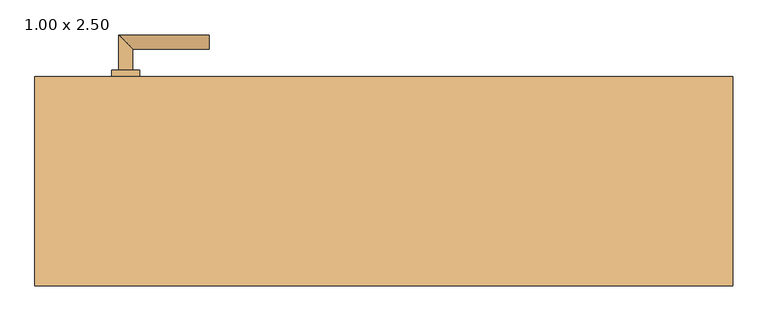
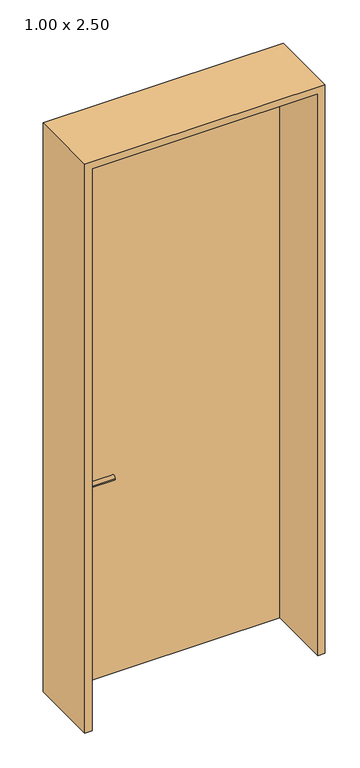
"""IFC4 building model written with IfcOpenShell, lengths in millimetres: door geometry, Drehflügel 1-flg - Blockzarge : 1.00 x 2.50."""

from ifc_helpers import new_model, si_unit, point, frame, frame_2d, origin, place, context, project, spatial, polyline, circle_curve, ellipse_curve, trimmed, segment, composite_curve, outline, extrude, source, transform, mapped, element, save
from ifc_brep_helpers import plane_surface, cylinder_surface, advanced_brep


def door_1_00_x_2_50_427c85ad(model_context):
    return source(origin(), model_context, "Body", "SolidModel", [
        advanced_brep(
        [(-360.0, 129.4346141, 1000.0), (-380.0, 129.4346141, 1000.0), (-360.0, 99.4346141, 1000.0), (-380.0, 79.4346141, 1000.0), (-250.0, 99.4346141, 1000.0), (-250.0, 79.4346141, 1000.0)],
        [
            (0, 1, circle_curve(frame((-370.0, 129.4346141, 1000.0), z_axis=(0.0, 1.0, 0.0), x_axis=(-1.0, 0.0, 0.0)), 10.0)),
            (1, 0, circle_curve(frame((-370.0, 129.4346141, 1000.0), z_axis=(0.0, 1.0, 0.0), x_axis=(-1.0, 0.0, 0.0)), 10.0)),
            (0, 2),
            (2, 3, ellipse_curve(frame((-370.0, 89.4346141, 1000.0), z_axis=(-0.7071067811865686, 0.7071067811865265, 0.0), x_axis=(0.7071067811865264, 0.7071067811865687, 0.0)), 14.1421356, 10.0)),
            (3, 1),
            (3, 2, ellipse_curve(frame((-370.0, 89.4346141, 1000.0), z_axis=(-0.7071067811865686, 0.7071067811865265, 0.0), x_axis=(0.7071067811865264, 0.7071067811865687, 0.0)), 14.1421356, 10.0)),
            (4, 5, circle_curve(frame((-250.0, 89.4346141, 1000.0), z_axis=(1.0, 0.0, 0.0), x_axis=(0.0, -1.0, 0.0)), 10.0)),
            (5, 4, circle_curve(frame((-250.0, 89.4346141, 1000.0), z_axis=(1.0, 0.0, 0.0), x_axis=(0.0, -1.0, 0.0)), 10.0)),
            (2, 4),
            (5, 3),
        ],
        [
            plane_surface(frame((-370.0, 129.4346141, -287.7526403), z_axis=(0.0, 1.0, 0.0), x_axis=(0.0, 0.0, 1.0))),
            cylinder_surface(frame((-370.0, 129.4346141, 1000.0), z_axis=(0.0, 1.0, 0.0), x_axis=(-1.0, 0.0, 0.0)), 10.0),
            plane_surface(frame((-250.0, 89.4346141, -287.7526403), z_axis=(1.0, 0.0, 0.0), x_axis=(0.0, 0.0, 1.0))),
            cylinder_surface(frame((-370.0, 89.4346141, 1000.0), z_axis=(-1.0, 0.0, 0.0), x_axis=(0.0, -1.0, 0.0)), 10.0),
        ],
        [
            (0, [[1, 2]]),
            (1, [[-1, 3, 4, 5]]),
            (1, [[-2, -5, 6, -3]]),
            (2, [[7, 8]]),
            (3, [[-4, 9, -8, 10]]),
            (3, [[-6, -10, -7, -9]]),
        ],
    ),
        advanced_brep(
        [(-360.0, 174.4346141, 1000.0), (-380.0, 174.4346141, 1000.0), (-360.0, 204.4346141, 1000.0), (-380.0, 224.4346141, 1000.0), (-250.0, 204.4346141, 1000.0), (-250.0, 224.4346141, 1000.0)],
        [
            (0, 1, circle_curve(frame((-370.0, 174.4346141, 1000.0), z_axis=(0.0, -1.0, 0.0), x_axis=(-1.0, 0.0, 0.0)), 10.0)),
            (1, 0, circle_curve(frame((-370.0, 174.4346141, 1000.0), z_axis=(0.0, -1.0, 0.0), x_axis=(-1.0, 0.0, 0.0)), 10.0)),
            (0, 2),
            (2, 3, ellipse_curve(frame((-370.0, 214.4346141, 1000.0), z_axis=(-0.7071067811865486, -0.7071067811865464, 0.0), x_axis=(0.7071067811865464, -0.7071067811865488, 0.0)), 14.1421356, 10.0)),
            (3, 1),
            (3, 2, ellipse_curve(frame((-370.0, 214.4346141, 1000.0), z_axis=(-0.7071067811865486, -0.7071067811865464, 0.0), x_axis=(0.7071067811865464, -0.7071067811865488, 0.0)), 14.1421356, 10.0)),
            (4, 5, circle_curve(frame((-250.0, 214.4346141, 1000.0), z_axis=(1.0, 0.0, 0.0), x_axis=(0.0, 1.0, 0.0)), 10.0)),
            (5, 4, circle_curve(frame((-250.0, 214.4346141, 1000.0), z_axis=(1.0, 0.0, 0.0), x_axis=(0.0, 1.0, 0.0)), 10.0)),
            (2, 4),
            (5, 3),
        ],
        [
            plane_surface(frame((-370.0, 174.4346141, -287.7526403), z_axis=(0.0, -1.0, 0.0), x_axis=(0.0, 0.0, 1.0))),
            cylinder_surface(frame((-370.0, 174.4346141, 1000.0), z_axis=(0.0, -1.0, 0.0), x_axis=(-1.0, 0.0, 0.0)), 10.0),
            plane_surface(frame((-250.0, 214.4346141, -287.7526403), z_axis=(1.0, 0.0, 0.0), x_axis=(0.0, 0.0, 1.0))),
            cylinder_surface(frame((-370.0, 214.4346141, 1000.0), z_axis=(-1.0, 0.0, 0.0), x_axis=(0.0, 1.0, 0.0)), 10.0),
        ],
        [
            (0, [[1, 2]]),
            (1, [[-1, 3, 4, 5]]),
            (1, [[-2, -5, 6, -3]]),
            (2, [[7, 8]]),
            (3, [[-4, 9, -8, 10]]),
            (3, [[-6, -10, -7, -9]]),
        ],
    ),
        extrude(outline(composite_curve([segment(trimmed(circle_curve(frame_2d((1000.0, -370.0)), 20.0), [point((1000.0, -350.0))], [point((1000.0, -390.0))], False, "CARTESIAN"), True, "CONTINUOUS"), segment(trimmed(circle_curve(frame_2d((1000.0, -370.0)), 20.0), [point((1000.0, -390.0))], [point((1000.0, -350.0))], False, "CARTESIAN"), True, "CONTINUOUS")], self_intersect=False)), frame((0.0, 129.4346141, 0.0), z_axis=(0.0, 1.0, 0.0), x_axis=(0.0, 0.0, 1.0)), (0.0, 0.0, 1.0), 10.0),
        extrude(outline(composite_curve([segment(trimmed(circle_curve(frame_2d((1000.0, -370.0)), 20.0), [point((1000.0, -350.0))], [point((1000.0, -390.0))], False, "CARTESIAN"), True, "CONTINUOUS"), segment(trimmed(circle_curve(frame_2d((1000.0, -370.0)), 20.0), [point((1000.0, -390.0))], [point((1000.0, -350.0))], False, "CARTESIAN"), True, "CONTINUOUS")], self_intersect=False)), frame((0.0, 164.4346141, 0.0), z_axis=(0.0, 1.0, 0.0), x_axis=(0.0, 0.0, 1.0)), (0.0, 0.0, 1.0), 10.0),
        extrude(outline(polyline([(2600.0, 500.0), (2600.0, -500.0), (100.0, -500.0), (100.0, -470.0), (2570.0, -470.0), (2570.0, 470.0), (100.0, 470.0), (100.0, 500.0), (2600.0, 500.0)])), frame((0.0, -135.5653859, 0.0), z_axis=(0.0, 1.0, 0.0), x_axis=(0.0, 0.0, 1.0)), (0.0, 0.0, 1.0), 300.0),
        extrude(outline(polyline([(470.0, 164.4346141), (470.0, 139.4346141), (-470.0, 139.4346141), (-470.0, 164.4346141), (470.0, 164.4346141)])), frame((0.0, 0.0, 100.0), z_axis=(0.0, 0.0, 1.0), x_axis=(1.0, 0.0, 0.0)), (0.0, 0.0, 1.0), 2470.0),
    ])


if __name__ == "__main__":
    model = new_model("IFC4")
    model_context = context("Model", 3, world=origin())
    ifc_project = project(units=[si_unit("LENGTHUNIT", "METRE", prefix="MILLI")], contexts=[model_context])
    site = spatial("IfcSite", under=ifc_project)
    building = spatial("IfcBuilding", under=site)
    placement = place(None, origin())
    door_1_00_x_2_50_shape = door_1_00_x_2_50_427c85ad(model_context)
    element("IfcDoor", 1, ObjectType="Drehflügel 1-flg - Blockzarge : 1.00 x 2.50", at=placement, inside=building, context=model_context, shape_type="MappedRepresentation", body=[
        mapped(door_1_00_x_2_50_shape, transform((0.0, 0.0, 0.0), x_axis=(1.0, 0.0, 0.0), y_axis=(0.0, 1.0, 0.0), z_axis=(0.0, 0.0, 1.0))),
    ])
    save(model, "model.ifc")

# Revit data of these elements
# Type "Drehflügel 1-flg - Blockzarge : 1.00 x 2.50"
#   Type Mark = "23"
#   Operation = "SingleSwingRight"
#   Keynote = "16.03"
#   Visual Light Transmittance = 0.9
#   Solar Heat Gain Coefficient = 0.86
#   Heat Transfer Coefficient (U) = 5.5617 W/(m²·K)
#   Rough Width = 1.000 m
#   Stärke Futter = 0.030 m
#   Rough Height [instance default] = 2.600 m
#   Höhe Türgriff = 0.900 m
#   Height = 2.500 m
#   Fußbodenaufbau [instance default] = 0.100 m
#   Width = 1.000 m
#   Sichtbarkeit Sturzlinien [instance default] = yes
#   Türgriff auswählen [instance default] = element 420047
#   Türgriff [instance default] = none
#   Türflügel [instance default] = none
#   Rahmen/Pfosten [instance default] = none
#   Construction Type Id = ""
#   Function = (empty or 0)
#   Wall Closure = (empty or 0)
#   Analytic Construction = (empty or 0)
# Element 1 (IfcDoor, "Drehflügel 1-flg - Blockzarge : 1.00 x 2.50")
#   Materials on its faces: "Metall - Chrom", "Holz - Birke"
# Materials
#   "Metall - Chrom": class "Metall", colour RGB 247 247 247, transparency 0, Cost = 0
#   "Holz - Birke": class "Holz", colour RGB 213 164 103, transparency 0, Cost = 0
